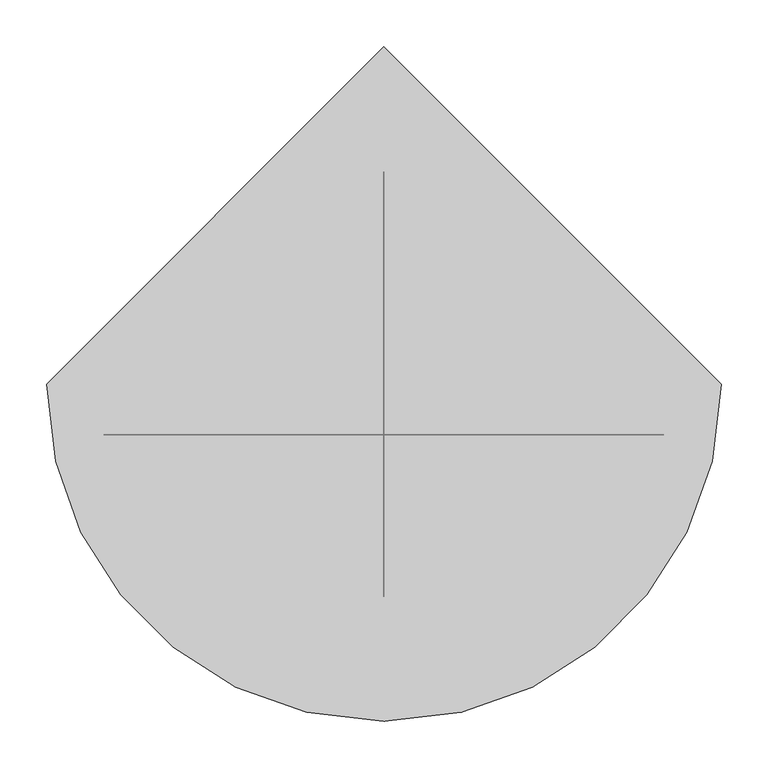
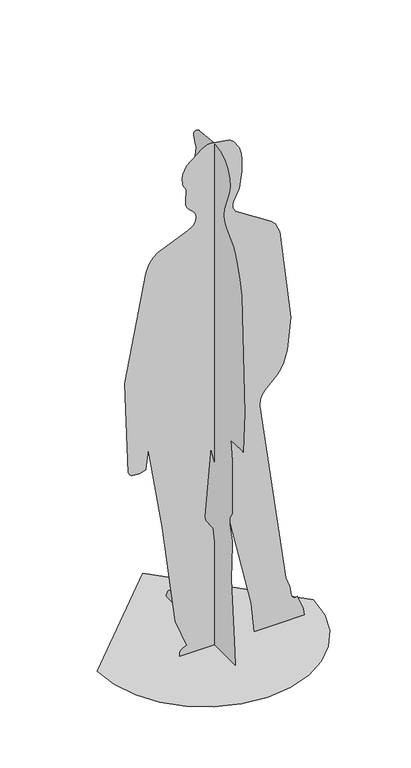
"""IFC4 building model written with IfcOpenShell, lengths in millimetres: proxy geometry, alex 23800 : alex 23800."""

import ifcopenshell
import ifcopenshell.guid

model = None  # the IFC model being written
_history = None  # IfcOwnerHistory: only IFC2X3 demands one
_inside = {}  # id of a spatial element -> (the spatial element, [elements in it])
_under = {}  # id of a project, library or spatial element -> (it, [spatial elements below it])
_declared = {}  # id of a project -> (the project, [libraries it declares])
_typed = {}  # id of a type object -> (the type object, [elements of that type])
_made_of = {}  # id of a material, layer set ... -> (it, [elements and type objects made of it])


def new_model(schema):
    """Start an empty IFC model of exactly this schema.

    Asked for "IFC4X3", IfcOpenShell would pick the latest addendum, in which some entities
    have other attributes; the version numbers below select the first issue.
    IFC2X3 requires an IfcOwnerHistory on every rooted entity: one is made here for all.
    """
    global model, _history
    if schema == "IFC4X3":
        model = ifcopenshell.file(schema_version=(4, 3, 0, 0))
    else:
        model = ifcopenshell.file(schema=schema)
    _inside.clear()
    _under.clear()
    _declared.clear()
    _typed.clear()
    _made_of.clear()
    _history = None
    if model.schema == "IFC2X3":
        org = make("IfcOrganization", Name="unknown")
        user = make(
            "IfcPersonAndOrganization",
            ThePerson=make("IfcPerson", FamilyName="unknown"),
            TheOrganization=org,
        )
        app = make(
            "IfcApplication",
            ApplicationDeveloper=org,
            Version="unknown",
            ApplicationFullName="unknown",
            ApplicationIdentifier="unknown",
        )
        _history = make(
            "IfcOwnerHistory",
            OwningUser=user,
            OwningApplication=app,
            ChangeAction="ADDED",
            CreationDate=0,
        )
    return model


def make(cls, **values):
    """One entity of the class cls with the attributes given. An attribute that is None is left unset."""
    return model.create_entity(
        cls, **{name: value for name, value in values.items() if value is not None}
    )


def rooted(cls, **values):
    """An entity with a GlobalId (a new one), such as an element, a storey or a relation."""
    return make(cls, GlobalId=ifcopenshell.guid.new(), OwnerHistory=_history, **values)


def si_unit(unit_type, name, prefix=None):
    """IfcSIUnit, for example si_unit("LENGTHUNIT", "METRE", prefix="MILLI")."""
    return make("IfcSIUnit", UnitType=unit_type, Prefix=prefix, Name=name)


def assignment(units):
    """IfcUnitAssignment: the units of a project."""
    return None if units is None else make("IfcUnitAssignment", Units=units)


def point(xyz):
    """IfcCartesianPoint."""
    return None if xyz is None else make("IfcCartesianPoint", Coordinates=xyz)


def direction(xyz):
    """IfcDirection."""
    return None if xyz is None else make("IfcDirection", DirectionRatios=xyz)


def frame(location, z_axis=None, x_axis=None):
    """IfcAxis2Placement3D, a coordinate frame: its origin and axes. An axis left out is left unset."""
    return make(
        "IfcAxis2Placement3D",
        Location=point(location),
        Axis=direction(z_axis),
        RefDirection=direction(x_axis),
    )


def origin():
    """The frame at (0, 0, 0) with its axes left unset."""
    return frame((0.0, 0.0, 0.0))


def place(relative_to, where):
    """IfcLocalPlacement: puts the frame where relative to a parent placement (None: the world)."""
    return make(
        "IfcLocalPlacement", PlacementRelTo=relative_to, RelativePlacement=where
    )


def context(
    kind, dimensions, precision=None, world=None, true_north=None, identifier=None
):
    """IfcGeometricRepresentationContext, for example the 3D "Model" context."""
    return make(
        "IfcGeometricRepresentationContext",
        ContextIdentifier=identifier,
        ContextType=kind,
        CoordinateSpaceDimension=dimensions,
        Precision=precision,
        WorldCoordinateSystem=world,
        TrueNorth=true_north,
    )


def project(units=None, contexts=None):
    """IfcProject with its units and contexts."""
    return rooted(
        "IfcProject",
        Name="project",
        RepresentationContexts=contexts,
        UnitsInContext=assignment(units),
    )


def spatial(cls, under=None, at=None, **own):
    """A site, building, storey or space (cls), placed at a placement, below another one or the project."""
    s = rooted(cls, ObjectPlacement=at, **own)
    if under is not None:
        _under.setdefault(under.id(), (under, []))[1].append(s)
    return s


def point_list(points):
    """IfcCartesianPointList2D or 3D."""
    cls = (
        "IfcCartesianPointList2D" if len(points[0]) == 2 else "IfcCartesianPointList3D"
    )
    return make(cls, CoordList=points)


def triangles(points, corners, closed=None, point_numbers=None):
    """IfcTriangulatedFaceSet: each triangle names its three corners, points numbered from 1."""
    return make(
        "IfcTriangulatedFaceSet",
        Coordinates=point_list(points),
        Closed=closed,
        CoordIndex=corners,
        PnIndex=point_numbers,
    )


def shape(context_of_items, identifier, shape_type, items):
    """IfcShapeRepresentation: the items that make up one representation, for example the "Body"."""
    return make(
        "IfcShapeRepresentation",
        ContextOfItems=context_of_items,
        RepresentationIdentifier=identifier,
        RepresentationType=shape_type,
        Items=items,
    )


def source(mapping_origin, context_of_items, identifier, shape_type, items):
    """IfcRepresentationMap: a shape defined once, which mapped items show again and again."""
    return make(
        "IfcRepresentationMap",
        MappingOrigin=mapping_origin,
        MappedRepresentation=shape(context_of_items, identifier, shape_type, items),
    )


def transform(
    local_origin,
    x_axis=None,
    y_axis=None,
    z_axis=None,
    scale=None,
    scale2=None,
    scale3=None,
    uniform=True,
):
    """IfcCartesianTransformationOperator3D, or its non-uniform kind. x_axis, y_axis, z_axis: its Axis1, 2, 3."""
    if uniform:
        return make(
            "IfcCartesianTransformationOperator3D",
            Axis1=direction(x_axis),
            Axis2=direction(y_axis),
            LocalOrigin=point(local_origin),
            Scale=scale,
            Axis3=direction(z_axis),
        )
    return make(
        "IfcCartesianTransformationOperator3DnonUniform",
        Axis1=direction(x_axis),
        Axis2=direction(y_axis),
        LocalOrigin=point(local_origin),
        Scale=scale,
        Axis3=direction(z_axis),
        Scale2=scale2,
        Scale3=scale3,
    )


def mapped(mapping_source, mapping_target):
    """IfcMappedItem: shows the shape of a source again, moved by a transform."""
    return make(
        "IfcMappedItem", MappingSource=mapping_source, MappingTarget=mapping_target
    )


def made_of(thing, what):
    """Note that an element or type object is made of a material, layer set ...; save() writes the relation."""
    if what is not None:
        _made_of.setdefault(what.id(), (what, []))[1].append(thing)
    return thing


def element(
    cls,
    number,
    at=None,
    inside=None,
    cuts=None,
    type_object=None,
    material=None,
    context=None,
    identifier="Body",
    shape_type=None,
    held_by="IfcProductDefinitionShape",
    body=None,
    shapes=None,
    **own,
):
    """One element of the class cls, such as IfcWall. Its Tag is "e" and its number.

    at: its placement. inside: the storey or other place that contains it. cuts: it is an
    opening in that element (IfcRelVoidsElement). A single representation is given by context,
    identifier, shape_type and body (its items); several are given by shapes. held_by: the class
    of the entity that holds the representations. save() writes the other relations.
    """
    e = rooted(cls, Tag="e%d" % number, ObjectPlacement=at, **own)
    if body is not None:
        shapes = [shape(context, identifier, shape_type, body)]
    if shapes is not None:
        e.Representation = make(held_by, Representations=shapes)
    if inside is not None:
        _inside.setdefault(inside.id(), (inside, []))[1].append(e)
    if cuts is not None:
        rooted(
            "IfcRelVoidsElement", RelatingBuildingElement=cuts, RelatedOpeningElement=e
        )
    if type_object is not None:
        _typed.setdefault(type_object.id(), (type_object, []))[1].append(e)
    return made_of(e, material)


def aggregate(whole, parts):
    """IfcRelAggregates: a whole, such as a stair, and the parts it consists of."""
    return rooted("IfcRelAggregates", RelatingObject=whole, RelatedObjects=parts)


def save(model, path):
    """Write the relations noted so far, then the file.

    IfcRelAggregates (storeys below a building ...), IfcRelContainedInSpatialStructure (elements
    in a storey), IfcRelDefinesByType, IfcRelAssociatesMaterial and IfcRelDeclares: one each for
    every whole, place, type object, material and project.
    """
    for whole, parts in _under.values():
        aggregate(whole, parts)
    for where, things in _inside.values():
        rooted(
            "IfcRelContainedInSpatialStructure",
            RelatedElements=things,
            RelatingStructure=where,
        )
    for kind, things in _typed.values():
        rooted("IfcRelDefinesByType", RelatedObjects=things, RelatingType=kind)
    for what, things in _made_of.values():
        rooted("IfcRelAssociatesMaterial", RelatedObjects=things, RelatingMaterial=what)
    for by, libraries in _declared.values():
        rooted("IfcRelDeclares", RelatingContext=by, RelatedDefinitions=libraries)
    model.write(path)


def entourage_2e3e706b(model_context):
    return source(origin(), model_context, "Body", "Tessellation", [
        triangles([(-117.149826, -54.2192196, 0.0), (-117.1651776, -54.2192196, 5.9668874), (-116.2257182, -54.2192196, 11.2908329), (-114.1990069, -54.2192196, 16.0246146), (-110.9487965, -54.2192196, 20.2200526), (-106.3426369, -54.2192196, 23.9299256), (-92.5232224, -54.2192196, 30.1060089), (-131.4701638, -54.2192196, 129.0202679), (-175.160493, -54.2192196, 475.7580242), (-222.3821928, -54.2192196, 767.9406984), (-230.1656384, -54.2192196, 699.5134071), (-235.7141188, -54.2192196, 696.8034708), (-252.8135111, -54.2192196, 693.0705591), (-271.5672719, -54.2192196, 693.4227905), (-279.1847031, -54.2192196, 695.8179932), (-284.3598959, -54.2192196, 700.0603941), (-288.7942909, -54.2192196, 709.0155161), (-300.0380995, -54.2192196, 1027.779562), (-230.6060912, -54.2192196, 1391.1560738), (-226.4231343, -54.2192196, 1402.4037884), (-221.6912647, -54.2192196, 1413.4720081), (-216.4584809, -54.2192196, 1423.8837273), (-210.7698928, -54.2192196, 1433.1671722), (-204.6734626, -54.2192196, 1440.846936), (-189.6343552, -54.2192196, 1451.6253479), (-89.8842756, -54.2192196, 1494.9825851), (-71.747551, -54.2192196, 1507.2129433), (-63.0092944, -54.2192196, 1520.5333511), (-61.6725528, -54.2192196, 1534.6925159), (-63.8671908, -54.2192196, 1545.3268959), (-68.585621, -54.2192196, 1553.4059086), (-87.7951952, -54.2192196, 1572.0070988), (-92.5232224, -54.2192196, 1579.5592541), (-95.9145034, -54.2192196, 1589.6919205), (-97.2061397, -54.2192196, 1598.308255), (-95.4740416, -54.2192196, 1641.5380291), (-96.331938, -54.2192196, 1644.515609), (-97.9843898, -54.2192196, 1647.8886589), (-100.1204967, -54.2192196, 1651.4987583), (-102.4302848, -54.2192196, 1655.1874866), (-104.5999834, -54.2192196, 1658.7975861), (-106.3205724, -54.2192196, 1662.170636), (-107.2792258, -54.2192196, 1665.1483612), (-108.4230876, -54.2192196, 1683.4309662), (-105.9731918, -54.2192196, 1699.5698067), (-100.5907078, -54.2192196, 1713.7231579), (-92.9406569, -54.2192196, 1726.0522018), (-41.9073575, -54.2192196, 1768.6831753), (-23.8378028, -54.2192196, 1776.4340103), (-13.1083444, -54.2192196, 1778.0000484), (45.7765254, -54.2192196, 1768.297443), (52.0927142, -54.2192196, 1765.4942711), (63.2559182, -54.2192196, 1755.9912174), (81.7812909, -54.2192196, 1728.0616722), (88.745219, -54.2192196, 1704.6000229), (91.0789973, -54.2192196, 1685.137112), (90.9475373, -54.2192196, 1642.2940876), (81.6066376, -54.2192196, 1585.4628181), (62.4047392, -54.2192196, 1543.9670952), (60.537325, -54.2192196, 1533.9496834), (60.9470838, -54.2192196, 1523.4841885), (69.4089674, -54.2192196, 1508.7943874), (187.9492836, -54.2192196, 1431.6201736), (202.6112339, -54.2192196, 1417.2355865), (217.8863916, -54.2192196, 1383.1912983), (254.1089989, -54.2192196, 1069.0535688), (242.364258, -54.2192196, 957.3563169), (229.1733843, -54.2192196, 912.5566532), (220.0532106, -54.2192196, 895.7643642), (208.0071618, -54.2192196, 880.6840347), (194.42189, -54.2192196, 866.7791422), (180.6849923, -54.2192196, 853.5153442), (168.1831209, -54.2192196, 840.3571358), (158.3057987, -54.2192196, 826.7670496), (152.4387149, -54.2192196, 812.2106707), (150.4446415, -54.2192196, 791.5933245), (238.0268047, -54.2192196, 154.0623804), (251.6370204, -54.2192196, 116.8321946), (256.996468, -54.2192196, 85.1121104), (259.9472872, -54.2192196, 78.4667766), (263.4038167, -54.2192196, 74.733874), (267.3257794, -54.2192196, 73.2493489), (271.6699546, -54.2192196, 73.3510687), (276.3951023, -54.2192196, 74.375938), (297.1717229, -54.2192196, 23.3148105), (300.0371367, -54.2192196, 0.0), (131.8280998, -54.2192196, 0.0), (122.3288704, -54.2192196, 103.0617143), (-12.8367732, -54.2192196, 700.0603941), (-32.6518678, -54.2192196, 465.9114232), (-30.5455124, -54.2192196, 452.1476558), (-28.5399163, -54.2192196, 446.8956871), (-9.3111464, -54.2192196, 418.9977533), (-6.9341794, -54.2192196, 413.7803392), (0.9020383, -54.2192196, 348.2760163), (3.9440186, -54.2192196, 338.8305536), (7.6318198, -54.2192196, 329.4100167), (11.5067468, -54.2192196, 320.0537564), (15.1043435, -54.2192196, 310.8021046), (17.965916, -54.2192196, 301.6953567), (20.1922245, -54.2192196, 275.8289304), (9.4637256, -54.2192196, 194.8220472), (10.7735997, -54.2192196, 177.672767), (25.5305637, -54.2192196, 136.3536502), (26.3020941, -54.2192196, 0.0), (0.0, -171.2567705, 45.1949975), (0.0, -150.8745481, 290.639618), (0.0, -156.0132787, 413.7064339), (0.0, -155.0152837, 426.2860439), (0.0, -142.9452446, 479.8709636), (0.0, -142.1842718, 491.5446696), (0.0, -143.2100995, 503.0207133), (0.0, -144.047839, 505.2451052), (0.0, -145.7118181, 508.1738508), (0.0, -147.8757485, 511.5296053), (0.0, -150.2143322, 515.036041), (0.0, -152.400327, 518.4148682), (0.0, -154.109416, 521.3887055), (0.0, -155.0152837, 523.6802808), (0.0, -156.6389491, 713.2963594), (0.0, -149.1126916, 780.4474205), (0.0, -210.0425026, 781.4050655), (0.0, -219.9447689, 780.4474205), (0.0, -227.6802342, 923.8398308), (0.0, -210.5088804, 1326.6335587), (0.0, -200.0250727, 1381.4668396), (0.0, -183.9208231, 1432.731443), (0.0, -173.3612024, 1455.0204895), (0.0, -160.9178849, 1474.0122082), (0.0, -124.7336655, 1511.6876701), (0.0, -116.986691, 1522.764465), (0.0, -111.1138482, 1535.6011814), (0.0, -107.7935748, 1550.7469139), (0.0, -109.4844237, 1573.6183376), (0.0, -138.1807553, 1647.6468132), (0.0, -144.3654704, 1674.2838501), (0.0, -143.232173, 1701.9783806), (0.0, -131.4049152, 1730.7792389), (0.0, -113.8084512, 1751.5885792), (0.0, -93.3149074, 1763.9963974), (0.0, -70.4587898, 1769.8088333), (0.0, -45.7765254, 1770.8327534), (0.0, 33.8705797, 1763.2439724), (0.0, 35.8723357, 1763.9599171), (0.0, 40.3067194, 1762.4466373), (0.0, 46.2419403, 1759.1397171), (0.0, 52.7442914, 1754.4731415), (0.0, 58.882952, 1748.8852558), (0.0, 63.7242081, 1742.8090279), (0.0, 66.3353223, 1736.6819309), (0.0, 66.7661872, 1728.2947975), (0.0, 65.1444384, 1720.0201572), (0.0, 62.192661, 1712.2874897), (0.0, 55.1980298, 1700.1665726), (0.0, 51.5783606, 1695.362796), (0.0, 72.2379144, 1580.2608101), (0.0, 61.7953832, 1563.4866886), (0.0, 54.5483692, 1508.478709), (0.0, -4.4967569, 1482.8666096), (0.0, 4.8441379, 1466.163414), (0.0, 131.2648075, 892.5976244), (0.0, 131.4039524, 884.7393105), (0.0, 130.533584, 877.3195599), (0.0, 128.9799633, 870.382556), (0.0, 127.06649, 863.9703747), (0.0, 125.1175083, 858.1292341), (0.0, 123.4573807, 852.9002655), (0.0, 122.4104424, 848.3277248), (0.0, 121.9344722, 836.2039009), (0.0, 123.662737, 824.5599169), (0.0, 138.1893939, 779.9867655), (0.0, 140.1191817, 768.6412371), (0.0, 134.7798818, 638.2851677), (0.0, 137.1673996, 618.1236803), (0.0, 142.9922621, 588.3899938), (0.0, 150.2623125, 530.9436092), (0.0, 150.5262045, 510.8147143), (0.0, 148.9725838, 491.2155109), (0.0, 104.741045, 115.2804997), (0.0, 107.6544391, 83.9308235), (0.0, 113.0014147, 72.9595455), (0.0, 123.907435, 63.6781489), (0.0, 138.4753594, 55.956123), (0.0, 154.8099183, 49.6658456), (0.0, 171.0159059, 44.676806), (0.0, 185.196145, 40.8613776), (0.0, 195.4573101, 38.0900079), (0.0, 202.9931691, 35.5086429), (0.0, 208.9821204, 32.4772168), (0.0, 213.7648408, 28.6934543), (0.0, 217.6848777, 23.8550755), (0.0, 221.0819088, 17.6607589), (0.0, 224.3004623, 9.8101468), (0.0, 227.6802342, 0.0), (0.0, -172.9495269, 0.0), (-361.2442655, 0.0, 0.0), (-351.6941943, -82.7735268, 0.0), (-324.4958181, -158.787528, 0.0), (-281.8265113, -225.8636845, 0.0), (-225.8646292, -281.8265113, 0.0), (-158.787528, -324.4948371, 0.0), (-82.7735268, -351.6941943, 0.0), (0.0, -361.2442655, 0.0), (82.7735268, -351.6941943, 0.0), (158.787528, -324.4958181, 0.0), (225.8646292, -281.8265113, 0.0), (281.8265113, -225.8636845, 0.0), (324.4958181, -158.787528, 0.0), (351.6941943, -82.7735268, 0.0), (361.2442655, 0.0, 0.0), (0.0, 361.2442655, 0.0)], [[85, 86, 87], [105, 1, 2], [105, 2, 3], [105, 3, 4], [105, 4, 5], [105, 5, 6], [105, 6, 7], [85, 87, 88], [104, 105, 7], [104, 7, 8], [103, 104, 8], [102, 103, 8], [102, 8, 9], [101, 102, 9], [100, 101, 9], [99, 100, 9], [98, 99, 9], [97, 98, 9], [96, 97, 9], [95, 96, 9], [94, 95, 9], [93, 94, 9], [92, 93, 9], [91, 92, 9], [90, 91, 9], [90, 9, 10], [89, 90, 10], [83, 84, 85], [10, 11, 12], [10, 12, 13], [10, 13, 14], [10, 14, 15], [10, 15, 16], [10, 16, 17], [10, 17, 18], [89, 10, 18], [89, 18, 19], [89, 19, 20], [89, 20, 21], [89, 21, 22], [89, 22, 23], [89, 23, 24], [89, 24, 25], [89, 25, 26], [89, 26, 27], [89, 27, 28], [82, 83, 85], [82, 85, 88], [81, 82, 88], [80, 81, 88], [79, 80, 88], [78, 79, 88], [77, 78, 88], [76, 77, 88], [76, 88, 89], [76, 89, 28], [75, 76, 28], [74, 75, 28], [73, 74, 28], [72, 73, 28], [71, 72, 28], [70, 71, 28], [69, 70, 28], [68, 69, 28], [67, 68, 28], [66, 67, 28], [65, 66, 28], [64, 65, 28], [63, 64, 28], [62, 63, 28], [61, 62, 28], [61, 28, 29], [60, 61, 29], [59, 60, 29], [59, 29, 30], [59, 30, 31], [58, 59, 31], [57, 58, 31], [57, 31, 32], [57, 32, 33], [57, 33, 34], [57, 34, 35], [57, 35, 36], [56, 57, 36], [56, 36, 37], [55, 56, 37], [54, 55, 37], [53, 54, 37], [52, 53, 37], [51, 52, 37], [50, 51, 37], [49, 50, 37], [48, 49, 37], [47, 48, 37], [47, 37, 38], [46, 47, 38], [45, 46, 38], [44, 45, 38], [43, 44, 38], [43, 38, 39], [43, 39, 40], [43, 40, 41], [43, 41, 42], [193, 194, 195], [192, 193, 195], [191, 192, 195], [190, 191, 195], [189, 190, 195], [188, 189, 195], [187, 188, 195], [186, 187, 195], [185, 186, 195], [184, 185, 195], [183, 184, 195], [182, 183, 195], [181, 182, 195], [181, 195, 106], [180, 181, 106], [179, 180, 106], [122, 123, 124], [179, 106, 107], [178, 179, 107], [178, 107, 108], [178, 108, 109], [178, 109, 110], [178, 110, 111], [177, 178, 111], [177, 111, 112], [176, 177, 112], [175, 176, 112], [175, 112, 113], [174, 175, 113], [174, 113, 114], [174, 114, 115], [174, 115, 116], [173, 174, 116], [173, 116, 117], [173, 117, 118], [173, 118, 119], [173, 119, 120], [173, 120, 121], [172, 173, 121], [171, 172, 121], [170, 171, 121], [169, 170, 121], [168, 169, 121], [167, 168, 121], [157, 158, 159], [166, 167, 121], [165, 166, 121], [164, 165, 121], [163, 164, 121], [162, 163, 121], [161, 162, 121], [121, 122, 124], [160, 161, 121], [160, 121, 124], [160, 124, 125], [160, 125, 126], [160, 126, 127], [160, 127, 128], [160, 128, 129], [159, 160, 129], [159, 129, 130], [159, 130, 131], [159, 131, 132], [157, 159, 132], [157, 132, 133], [157, 133, 134], [156, 157, 134], [155, 156, 134], [155, 134, 135], [155, 135, 136], [155, 136, 137], [155, 137, 138], [155, 138, 139], [155, 139, 140], [155, 140, 141], [155, 141, 142], [155, 142, 143], [154, 155, 143], [153, 154, 143], [152, 153, 143], [151, 152, 143], [150, 151, 143], [149, 150, 143], [148, 149, 143], [147, 148, 143], [146, 147, 143], [145, 146, 143], [144, 145, 143], [210, 211, 196], [209, 210, 196], [209, 196, 197], [208, 209, 197], [208, 197, 198], [208, 198, 199], [207, 208, 199], [206, 207, 199], [206, 199, 200], [206, 200, 201], [206, 201, 202], [206, 202, 203], [206, 203, 204], [206, 204, 205]], closed=False),
    ])


if __name__ == "__main__":
    model = new_model("IFC4")
    model_context = context("Model", 3, world=origin())
    ifc_project = project(units=[si_unit("LENGTHUNIT", "METRE", prefix="MILLI")], contexts=[model_context])
    site = spatial("IfcSite", under=ifc_project)
    building = spatial("IfcBuilding", under=site)
    placement = place(None, origin())
    entourage_shape = entourage_2e3e706b(model_context)
    element("IfcBuildingElementProxy", 1, Name="alex 23800 : alex 23800", ObjectType="alex 23800 : alex 23800", at=placement, inside=building, context=model_context, shape_type="MappedRepresentation", body=[
        mapped(entourage_shape, transform((0.0, 0.0, 0.0), x_axis=(1.0, 0.0, 0.0), y_axis=(0.0, 1.0, 0.0), z_axis=(0.0, 0.0, 1.0))),
    ])
    save(model, "model.ifc")

# Revit data of these elements
# Type "alex 23800 : alex 23800"
#   built-in parameter 1005195 = "RPC-8-X9C2-NGU9-LXF5-4"
#   Height = 0
